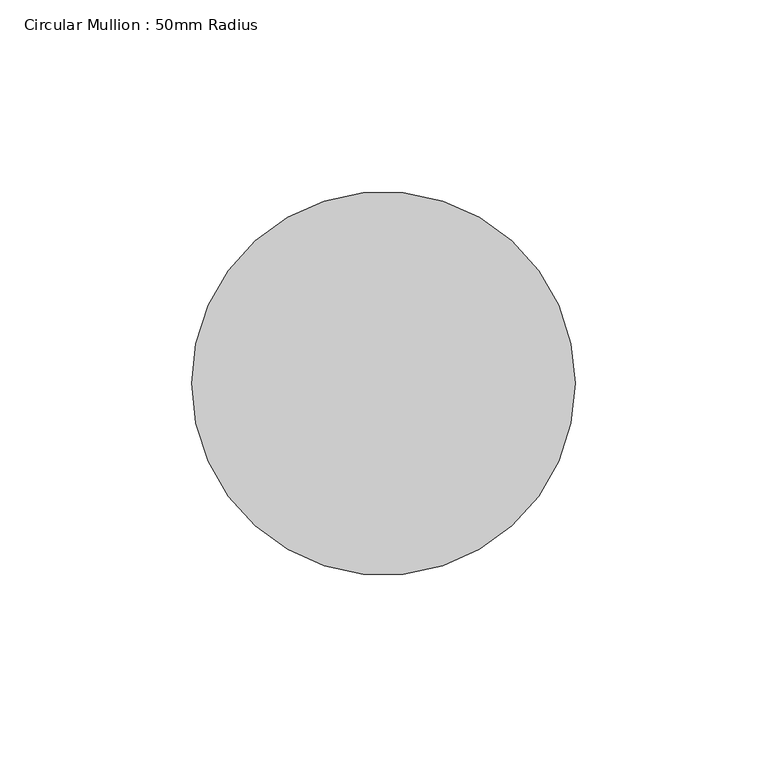
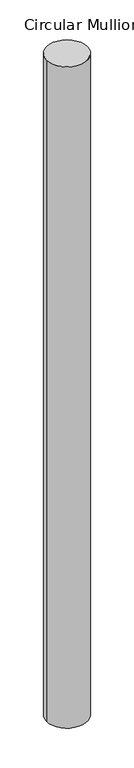
"""IFC4 building model written with IfcOpenShell, lengths in millimetres: member geometry, Circular Mullion : 50mm Radius."""

from ifc_helpers import new_model, si_unit, point, frame, origin, origin_2d, place, context, project, spatial, circle_curve, trimmed, segment, composite_curve, outline, extrude, source, transform, mapped, element, save


def circular_mullion_50mm_radius_34f998ff(model_context):
    return source(origin(), model_context, "Body", "SweptSolid", [
        extrude(outline(composite_curve([segment(trimmed(circle_curve(origin_2d(), 50.0), [point((50.0, 0.0))], [point((-50.0, 0.0))], False, "CARTESIAN"), True, "CONTINUOUS"), segment(trimmed(circle_curve(origin_2d(), 50.0), [point((-50.0, 0.0))], [point((50.0, 0.0))], False, "CARTESIAN"), True, "CONTINUOUS")], self_intersect=False)), frame((0.0, 0.0, -1708.9502931), z_axis=(0.0, 0.0, 1.0), x_axis=(1.0, 0.0, 0.0)), (0.0, 0.0, 1.0), 1708.9502931),
    ])


if __name__ == "__main__":
    model = new_model("IFC4")
    model_context = context("Model", 3, world=origin())
    ifc_project = project(units=[si_unit("LENGTHUNIT", "METRE", prefix="MILLI")], contexts=[model_context])
    site = spatial("IfcSite", under=ifc_project)
    building = spatial("IfcBuilding", under=site)
    placement = place(None, origin())
    circular_mullion_50mm_radius_shape = circular_mullion_50mm_radius_34f998ff(model_context)
    element("IfcMember", 1, ObjectType="Circular Mullion : 50mm Radius", at=placement, inside=building, context=model_context, shape_type="MappedRepresentation", body=[
        mapped(circular_mullion_50mm_radius_shape, transform((0.0, 0.0, 0.0), x_axis=(1.0, 0.0, 0.0), y_axis=(0.0, 1.0, 0.0), z_axis=(0.0, 0.0, 1.0))),
    ])
    save(model, "model.ifc")

# Revit data of these elements
# Type "Circular Mullion : 50mm Radius"
#   built-in parameter 1007350 = 0.164042 (stored number, unit not read)
# Element 1 (IfcMember, "Circular Mullion : 50mm Radius")
#   Materials on its faces: "Aluminium"
# Materials
#   "Aluminium": class "Metal", colour RGB 247 247 247, transparency 0, Description = "Aluminium 6061", Cost = 0
